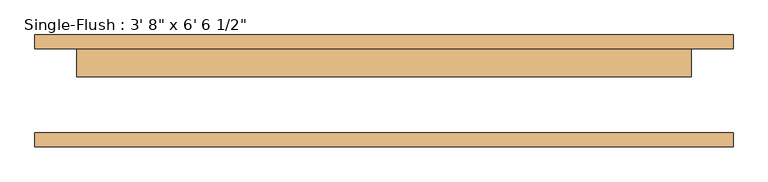
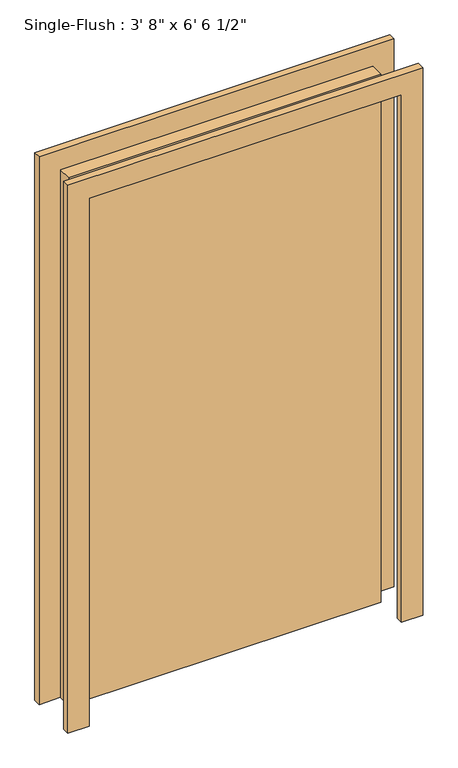
"""IFC4 building model written with IfcOpenShell, lengths in millimetres: door geometry."""

from ifc_helpers import new_model, si_unit, frame, origin, origin_with_axes, place, context, project, spatial, polyline, outline, extrude, source, transform, mapped, element, save


def door_d1072818(model_context):
    return source(origin(), model_context, "Body", "SweptSolid", [
        extrude(outline(polyline([(2070.1, -635.0), (0.0, -635.0), (0.0, -558.8), (1993.9, -558.8), (1993.9, 558.8), (0.0, 558.8), (0.0, 635.0), (2070.1, 635.0), (2070.1, -635.0)])), frame((0.0, 76.2, 0.0), z_axis=(0.0, 1.0, 0.0), x_axis=(0.0, 0.0, 1.0)), (0.0, 0.0, 1.0), 25.4),
        extrude(outline(polyline([(2070.1, 635.0), (2070.1, -635.0), (0.0, -635.0), (0.0, -558.8), (1993.9, -558.8), (1993.9, 558.8), (0.0, 558.8), (0.0, 635.0), (2070.1, 635.0)])), frame((0.0, -101.6, 0.0), z_axis=(0.0, 1.0, 0.0), x_axis=(0.0, 0.0, 1.0)), (0.0, 0.0, 1.0), 25.4),
        extrude(outline(polyline([(558.8, 25.4), (-558.8, 25.4), (-558.8, 76.2), (558.8, 76.2), (558.8, 25.4)])), origin_with_axes(), (0.0, 0.0, 1.0), 1993.9),
    ])


if __name__ == "__main__":
    model = new_model("IFC4")
    model_context = context("Model", 3, world=origin())
    ifc_project = project(units=[si_unit("LENGTHUNIT", "METRE", prefix="MILLI")], contexts=[model_context])
    site = spatial("IfcSite", under=ifc_project)
    building = spatial("IfcBuilding", under=site)
    placement = place(None, origin())
    door_shape = door_d1072818(model_context)
    element("IfcDoor", 1, ObjectType="Single-Flush : 3' 8\" x 6' 6 1/2\"", at=placement, inside=building, context=model_context, shape_type="MappedRepresentation", body=[
        mapped(door_shape, transform((0.0, 0.0, 0.0), x_axis=(1.0, 0.0, 0.0), y_axis=(0.0, 1.0, 0.0), z_axis=(0.0, 0.0, 1.0))),
    ])
    save(model, "model.ifc")

# Revit data of these elements
# Type "Single-Flush : 3' 8\" x 6' 6 1/2\""
#   Type Mark = "10"
#   Assembly Code = "C1020"
#   Thickness = 0' - 2"
#   Height = 6' - 6 1/2"
#   Trim Projection Ext = 0' - 1"
#   Trim Projection Int = 0' - 1"
#   Trim Width = 0' - 3"
#   Width = 3' - 8"
#   Door Material = Door - Panel
#   Frame Material = Door - Frame
#   Function = (empty or 0)
#   Wall Closure = (empty or 0)
# Element 1 (IfcDoor, "Single-Flush : 3' 8\" x 6' 6 1/2\"")
#   Materials on its faces: "Door - Frame", "Door - Panel"
# Materials
#   "Door - Panel": class "Wood", colour RGB 114 82 51, transparency 0
#   "Door - Frame": class "Miscellaneous", colour RGB 153 76 43, transparency 0
